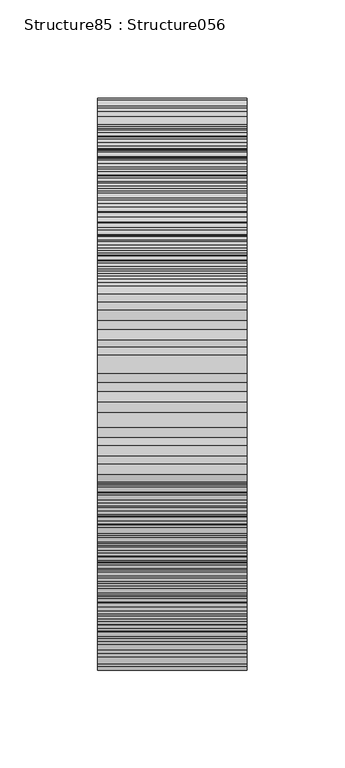
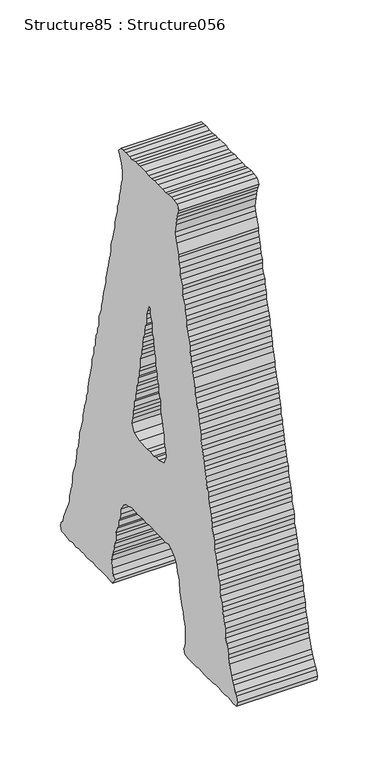
"""IFC4 building model written with IfcOpenShell, lengths in millimetres: proxy geometry, Structure85 : Structure056."""

from ifc_helpers import new_model, si_unit, frame, origin, place, context, project, spatial, polyline, outline, extrude, source, transform, mapped, element, save


def structure85_structure056_11b97279(model_context):
    return source(origin(), model_context, "Body", "SweptSolid", [
        extrude(outline(polyline([(278723.5580042, 3818.8310229), (278723.5580042, 3814.7296538), (278724.7389931, 3811.2043377), (278727.0785064, 3805.9476534), (278727.0785064, 3801.8462843), (278727.6802331, 3795.960595), (278730.0197465, 3791.8865042), (278730.0197465, 3787.7867397), (278732.3608644, 3783.0868532), (278732.9401266, 3777.8285642), (278732.9401266, 3773.11905), (278735.27964, 3769.6274306), (278735.27964, 3763.759392), (278737.0398911, 3759.6596275), (278738.8017469, 3755.559863), (278738.8017469, 3750.8583719), (278739.9602713, 3746.1745313), (278742.3222491, 3737.400554), (278743.503238, 3732.1149867), (278744.6617625, 3727.4311462), (278745.844356, 3723.3313817), (278745.844356, 3718.6571688), (278747.5821427, 3713.3555556), (278748.1614049, 3709.2718371), (278749.9441205, 3704.5879966), (278751.1026449, 3701.0723082), (278751.6819072, 3695.786741), (278753.4437629, 3690.512406), (278753.4437629, 3685.8285655), (278754.6247518, 3682.8857208), (278755.7832762, 3677.6274319), (278757.5435274, 3672.9435914), (278759.3037785, 3668.8261762), (278759.8846453, 3664.1423357), (278760.486372, 3660.0682449), (278761.0656342, 3654.1841602), (278763.4051476, 3650.1004418), (278763.9844098, 3645.9830266), (278764.5861365, 3641.2991861), (278765.1653987, 3636.0408972), (278766.3239232, 3631.915459), (278768.1082434, 3627.8397636), (278769.84603, 3622.555801), (278771.027019, 3617.2718384), (278771.027019, 3613.772196), (278771.6062812, 3607.8961343), (278773.3665323, 3604.3964919), (278774.5475212, 3600.2967274), (278775.7076503, 3595.5872132), (278776.309377, 3589.7544759), (278777.4679014, 3586.2115092), (278781.5676659, 3577.4535778), (278783.9087838, 3572.1423369), (278785.669035, 3568.6426945), (278786.8500239, 3563.366755), (278789.7704041, 3560.441561), (278790.951393, 3556.3417965), (278789.1895372, 3551.6675836), (278784.5105105, 3551.6675836), (278779.8074148, 3551.0658569), (278775.7076503, 3550.4833855), (278770.4477567, 3551.6675836), (278765.1653987, 3550.4833855), (278760.486372, 3551.6675836), (278756.9642652, 3551.0658569), (278751.1026449, 3551.6675836), (278747.5821427, 3551.0658569), (278741.7205224, 3551.0658569), (278737.620758, 3551.6675836), (278733.5193889, 3551.0658569), (278728.8387576, 3551.0658569), (278724.1597308, 3551.6675836), (278714.7760038, 3551.6675836), (278710.096977, 3551.0658569), (278704.814619, 3550.4833855), (278701.2941168, 3556.3417965), (278704.2353568, 3559.2669905), (278705.995608, 3565.1254015), (278706.5748702, 3572.7440636), (278704.814619, 3578.6104977), (278703.0543679, 3582.7102621), (278702.4751057, 3587.3860796), (278701.8958435, 3592.0955938), (278699.532261, 3596.7698067), (278699.532261, 3601.4536473), (278698.9529988, 3604.9709403), (278697.7944744, 3610.2292293), (278695.4324966, 3613.772196), (278694.8532343, 3619.6145609), (278693.0929832, 3622.555801), (278691.9328542, 3627.8397636), (278691.9328542, 3633.0980525), (278687.2538274, 3639.5405396), (278683.7092561, 3643.0578326), (278676.6891114, 3644.8245022), (278673.1686092, 3645.9830266), (278667.3294534, 3645.4262289), (278663.2072245, 3644.8245022), (278658.5265932, 3645.4262289), (278653.8459618, 3645.9830266), (278649.7461974, 3644.8245022), (278644.4638394, 3645.4262289), (278632.1613367, 3645.4262289), (278626.3013211, 3644.8245022), (278616.917594, 3644.8245022), (278612.2385673, 3645.9830266), (278605.7976848, 3642.4833842), (278601.6963157, 3638.9580681), (278598.7550757, 3633.0980525), (278597.5965513, 3627.2396415), (278595.8346955, 3622.555801), (278594.6537066, 3619.6145609), (278593.4951822, 3609.0723094), (278592.3141933, 3604.3964919), (278591.1556688, 3600.2967274), (278589.3954177, 3596.1953583), (278588.2128242, 3592.0955938), (278587.6335619, 3586.2115092), (278585.8733108, 3582.7102621), (278584.7147864, 3578.6104977), (278584.7147864, 3573.9266571), (278584.7147864, 3563.9412034), (278585.8733108, 3559.2669905), (278587.6335619, 3555.7416744), (278585.2940486, 3551.6675836), (278580.0116906, 3550.4833855), (278566.5506635, 3550.4833855), (278562.450899, 3551.6675836), (278557.168541, 3551.0658569), (278552.4670498, 3550.4833855), (278548.3881452, 3550.4833855), (278542.5040605, 3551.0658569), (278538.404296, 3551.0658569), (278533.7236647, 3551.6675836), (278529.6239002, 3551.6675836), (278524.9432689, 3550.4833855), (278519.6609109, 3550.4833855), (278514.9818842, 3551.6675836), (278509.6995262, 3551.0658569), (278506.1998838, 3550.4833855), (278500.3174037, 3551.0658569), (278499.1572747, 3555.1848766), (278500.9191304, 3560.441561), (278502.0776548, 3563.366755), (278505.5981571, 3568.6426945), (278507.3600128, 3572.1423369), (278509.120264, 3576.2693797), (278512.0390395, 3586.2115092), (278513.7992907, 3590.3289243), (278513.7992907, 3594.4286888), (278514.9818842, 3599.1125293), (278516.1404086, 3604.3964919), (278518.5023865, 3608.4705827), (278519.0816487, 3612.5976255), (278519.0816487, 3617.2718384), (278520.2401731, 3622.555801), (278522.0228887, 3627.2396415), (278522.5812911, 3632.5155811), (278523.76228, 3636.0408972), (278524.9432689, 3640.114988), (278526.6810556, 3645.4262289), (278527.8620445, 3650.6845178), (278527.8620445, 3655.3587307), (278529.0430334, 3659.4584952), (278531.3841513, 3663.5598643), (278531.3841513, 3668.8261762), (278533.1444025, 3673.5276674), (278533.7236647, 3677.0449604), (278535.4839158, 3682.8857208), (278536.6649047, 3686.4030139), (278536.6649047, 3691.0868544), (278537.2457716, 3695.2122926), (278538.404296, 3699.8881101), (278540.7662738, 3705.7545441), (278540.7662738, 3710.4560353), (278541.9247983, 3714.5301261), (278543.1057872, 3718.0554422), (278544.2867761, 3723.3313817), (278546.0261674, 3727.4311462), (278547.2071563, 3732.7167134), (278547.2071563, 3737.9750024), (278548.9674074, 3740.9162424), (278550.1259319, 3745.6000829), (278550.7276585, 3751.4424479), (278552.4670498, 3756.1423345), (278553.6480387, 3759.6596275), (278554.2273009, 3764.3611187), (278554.8290276, 3769.0176809), (278556.5668143, 3774.3032481), (278557.168541, 3777.8285642), (278558.9287921, 3783.0868532), (278558.9287921, 3788.3611881), (278560.0889212, 3791.8865042), (278561.8491723, 3797.1463977), (278562.450899, 3801.8462843), (278563.6094234, 3806.5317294), (278564.1886857, 3810.0474179), (278566.5506635, 3815.3313805), (278567.7107925, 3820.015221), (278568.8917814, 3824.1149855), (278568.8917814, 3829.374879), (278571.810557, 3837.6000817), (278572.9915459, 3842.8583706), (278573.5708081, 3846.9757858), (278575.3326639, 3851.6612309), (278575.3326639, 3856.9179152), (278577.092915, 3861.0192843), (278577.6721772, 3866.3032469), (278578.2514395, 3869.8189354), (278580.0116906, 3873.9203044), (278581.7735463, 3878.5784713), (278582.9320708, 3883.8881076), (278582.9320708, 3888.5623205), (278584.1130597, 3892.6636896), (278585.8733108, 3897.3475301), (278585.8733108, 3902.6314927), (278588.2128242, 3906.1487857), (278589.3954177, 3910.8310217), (278589.9746799, 3916.0909152), (278589.9746799, 3919.6066036), (278592.3141933, 3924.2888396), (278593.4951822, 3928.9919353), (278594.0744444, 3934.2758979), (278595.2554333, 3938.9517154), (278596.4155623, 3944.235678), (278596.4155623, 3947.1496398), (278599.9360646, 3956.5349715), (278601.1170535, 3961.794865), (278602.275578, 3965.8930249), (278600.5153268, 3974.7055128), (278599.3568024, 3979.9621971), (278598.7550757, 3983.4794902), (278597.5965513, 3987.5792547), (278595.2554333, 3991.6806238), (278598.7550757, 3996.390138), (278604.0374337, 3996.9645864), (278608.1371982, 3997.5486624), (278613.4195562, 3997.5486624), (278617.5193207, 3996.390138), (278622.8016787, 3996.9645864), (278630.4010856, 3996.9645864), (278635.6834436, 3997.5486624), (278640.9433371, 3996.390138), (278645.6448283, 3996.390138), (278650.3254596, 3997.5486624), (278659.7075821, 3997.5486624), (278663.8089512, 3996.9645864), (278667.3294534, 3997.5486624), (278672.589347, 3996.390138), (278677.2683737, 3996.390138), (278682.5507317, 3997.5486624), (278686.6521008, 3997.5486624), (278690.7518652, 3996.9645864), (278694.8532343, 3992.2614906), (278692.5121164, 3987.5792547), (278690.7518652, 3984.0635662), (278689.5933408, 3979.3781211), (278688.4123519, 3974.7055128), (278688.4123519, 3966.5043792), (278690.172603, 3962.3757319), (278691.3311275, 3957.1190475), (278691.9328542, 3952.435207), (278693.6947099, 3947.7337158), (278693.6947099, 3944.235678), (278694.8532343, 3938.3499888), (278696.6134855, 3934.8503464), (278696.6134855, 3929.5904528), (278698.3737366, 3924.8905662), (278700.1339877, 3919.6066036), (278701.2941168, 3915.5068392), (278701.2941168, 3910.8310217), (278702.4751057, 3906.1487857), (278703.6336301, 3902.6314927), (278704.814619, 3896.763454), (278706.5748702, 3893.822214), (278707.7558591, 3888.5623205), (278707.7558591, 3884.4609514), (278708.3367259, 3878.5784713), (278710.096977, 3875.0772243), (278710.6762393, 3870.4030114), (278711.8572282, 3866.3032469), (278713.0157526, 3861.0192843), (278714.1967415, 3856.9179152), (278715.9585973, 3851.6612309), (278715.9585973, 3846.9757858), (278717.6963839, 3841.6741725), (278718.2981106, 3838.1761347), (278720.0583618, 3833.4730389), (278720.637624, 3828.2163546), (278721.2168862, 3824.1149855), (278723.5580042, 3818.8310229)]), holes=[polyline([(278660.8661065, 3720.4158154), (278669.0672401, 3723.9154578), (278672.589347, 3730.9323932), (278671.4308225, 3736.7988273), (278670.248229, 3741.5003184), (278670.248229, 3744.9999608), (278668.4879779, 3750.3015741), (278668.4879779, 3755.559863), (278666.7277267, 3759.0595054), (278666.1484645, 3764.3611187), (278664.9674756, 3768.4432325), (278664.9674756, 3773.11905), (278662.6263576, 3777.8285642), (278662.6263576, 3783.0868532), (278660.8661065, 3786.0280932), (278660.2868443, 3790.7039107), (278659.1058554, 3795.4037973), (278658.5265932, 3804.7730829), (278656.766342, 3810.0474179), (278656.1870798, 3814.7296538), (278655.0044863, 3818.8310229), (278654.4252241, 3822.932392), (278653.8459618, 3828.790803), (278651.5064485, 3833.4730389), (278651.5064485, 3836.9919366), (278650.9047218, 3842.2758992), (278648.5652085, 3845.8012153), (278648.5652085, 3851.0595042), (278647.9843416, 3855.7353217), (278646.2240905, 3860.4432313), (278645.065566, 3865.1190488), (278643.2828505, 3864.5446004), (278643.2828505, 3860.4432313), (278642.124326, 3856.3161885), (278640.3624703, 3851.6612309), (278640.3624703, 3846.3772683), (278639.783208, 3842.2758992), (278637.4436947, 3837.6000817), (278637.4436947, 3832.8921721), (278636.841968, 3828.790803), (278635.6834436, 3824.1149855), (278634.5024547, 3819.4150989), (278633.9231924, 3813.5743386), (278633.3423256, 3810.0474179), (278631.5820745, 3805.9476534), (278631.5820745, 3800.6717138), (278629.2425611, 3795.4037973), (278629.2425611, 3790.7039107), (278628.0615722, 3786.0280932), (278626.3013211, 3782.5027771), (278625.7204542, 3777.2444882), (278625.7204542, 3772.5606477), (278625.1187276, 3767.8607611), (278623.3809409, 3763.759392), (278622.8016787, 3759.6596275), (278622.199952, 3754.9854146), (278619.8604386, 3750.8583719), (278620.4397009, 3744.9999608), (278619.2811764, 3740.9162424), (278618.0985829, 3736.7988273), (278616.917594, 3730.9323932), (278619.8604386, 3723.3313817), (278628.6408344, 3720.4158154), (278632.7405989, 3720.9726131), (278636.841968, 3719.8140887), (278642.124326, 3720.9726131), (278647.4050794, 3720.4158154), (278660.8661065, 3720.4158154)])]), frame((-59031.6926606, 0.0, 0.0), z_axis=(1.0, 0.0, 0.0), x_axis=(0.0, 1.0, 0.0)), (0.0, 0.0, 1.0), 76.2),
    ])


if __name__ == "__main__":
    model = new_model("IFC4")
    model_context = context("Model", 3, world=origin())
    ifc_project = project(units=[si_unit("LENGTHUNIT", "METRE", prefix="MILLI")], contexts=[model_context])
    site = spatial("IfcSite", under=ifc_project)
    building = spatial("IfcBuilding", under=site)
    placement = place(None, origin())
    structure85_structure056_shape = structure85_structure056_11b97279(model_context)
    element("IfcBuildingElementProxy", 1, Name="Structure85 : Structure056", ObjectType="Structure85 : Structure056", at=placement, inside=building, context=model_context, shape_type="MappedRepresentation", body=[
        mapped(structure85_structure056_shape, transform((0.0, 0.0, 0.0), x_axis=(1.0, 0.0, 0.0), y_axis=(0.0, 1.0, 0.0), z_axis=(0.0, 0.0, 1.0))),
    ])
    save(model, "model.ifc")

# Revit data of these elements
# Type "Structure85 : Structure056"
#   NameOverride = "Structure056"
# Element 1 (IfcBuildingElementProxy, "Structure85 : Structure056")
#   Materials on its faces: "BRUSHED ALUM. LETTERING"
# Materials
#   "BRUSHED ALUM. LETTERING": class "Unassigned", colour RGB 169 181 186, transparency 0, Cost = 0
